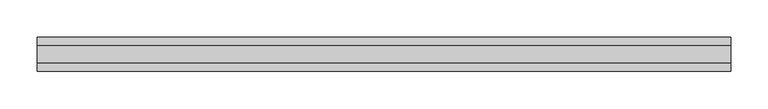
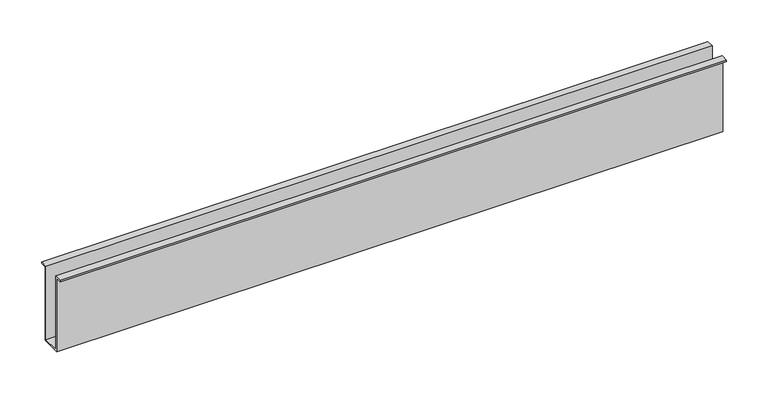
"""IFC4 building model written with IfcOpenShell, lengths in millimetres: railing geometry, ML_Perfil U de embutir4 : ML_Perfil U de embutir."""

from ifc_helpers import new_model, si_unit, frame, origin, place, context, project, spatial, polyline, outline, extrude, source, transform, mapped, element, save


def railing_24874f95(model_context):
    return source(origin(), model_context, "Body", "SweptSolid", [
        extrude(outline(polyline([(1832.4523952, 3702.0), (1832.4523952, 3594.0), (1856.4523952, 3594.0), (1856.4523952, 3702.0), (1866.9523952, 3702.0), (1866.9523952, 3700.0), (1858.4523952, 3700.0), (1858.4523952, 3592.0), (1830.4523952, 3592.0), (1830.4523952, 3700.0), (1821.9523952, 3700.0), (1821.9523952, 3702.0), (1832.4523952, 3702.0)])), frame((-12226.1487231, 0.0, 0.0), z_axis=(1.0, 0.0, 0.0), x_axis=(0.0, 1.0, 0.0)), (0.0, 0.0, 1.0), 925.0),
    ])


if __name__ == "__main__":
    model = new_model("IFC4")
    model_context = context("Model", 3, world=origin())
    ifc_project = project(units=[si_unit("LENGTHUNIT", "METRE", prefix="MILLI")], contexts=[model_context])
    site = spatial("IfcSite", under=ifc_project)
    building = spatial("IfcBuilding", under=site)
    placement = place(None, origin())
    railing_shape = railing_24874f95(model_context)
    element("IfcRailing", 1, ObjectType="ML_Perfil U de embutir4 : ML_Perfil U de embutir", at=placement, inside=building, context=model_context, shape_type="MappedRepresentation", body=[
        mapped(railing_shape, transform((0.0, 0.0, 0.0), x_axis=(1.0, 0.0, 0.0), y_axis=(0.0, 1.0, 0.0), z_axis=(0.0, 0.0, 1.0))),
    ])
    save(model, "model.ifc")

# Revit data of these elements
# Type "ML_Perfil U de embutir4 : ML_Perfil U de embutir"
#   ME_Compr [instance default] = 0.925 m
#   ME_Material Perfil [instance default] = .ALUMÍNIO COM PINTURA ELETROSTÁTICA BRANCA
# Element 1 (IfcRailing, "ML_Perfil U de embutir4 : ML_Perfil U de embutir")
#   Materials on its faces: ".ALUMÍNIO COM PINTURA ELETROSTÁTICA BRANCA"
# Materials
#   ".ALUMÍNIO COM PINTURA ELETROSTÁTICA BRANCA": class "CC_METAIS", colour RGB 241 241 241, transparency 0, Cost = 0
